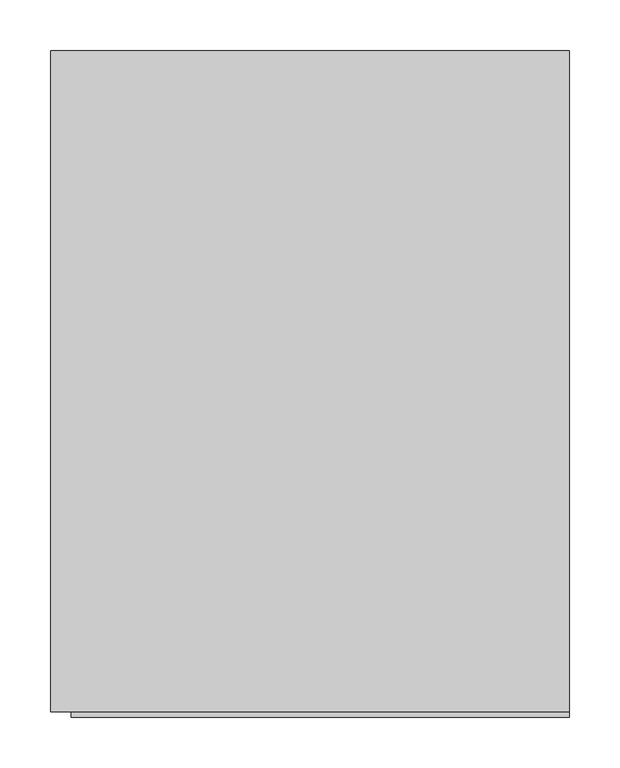
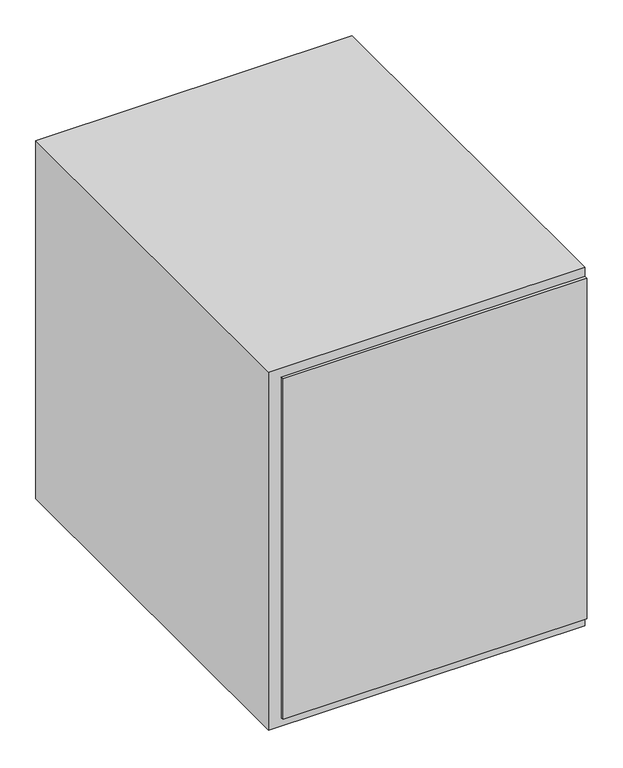
"""IFC4 building model written with IfcOpenShell, lengths in millimetres: proxy geometry, Тропик-30 : LNVx 45F."""

from ifc_helpers import new_model, si_unit, frame, origin, origin_with_axes, place, context, project, spatial, polyline, outline, extrude, source, transform, mapped, element, save


def mechanical_equipment_ab37a4de(model_context):
    return source(origin(), model_context, "Body", "SweptSolid", [
        extrude(outline(polyline([(255.0, -330.0), (-234.7800933, -330.0), (-234.7800933, -325.0), (255.0, -325.0), (255.0, -330.0)])), frame((0.0, 0.0, 14.5270889), z_axis=(0.0, 0.0, 1.0), x_axis=(1.0, 0.0, 0.0)), (0.0, 0.0, 1.0), 580.0),
        extrude(outline(polyline([(255.0, 325.0), (255.0, -325.0), (-255.0, -325.0), (-255.0, 325.0), (255.0, 325.0)])), origin_with_axes(), (0.0, 0.0, 1.0), 610.0),
    ])


if __name__ == "__main__":
    model = new_model("IFC4")
    model_context = context("Model", 3, world=origin())
    ifc_project = project(units=[si_unit("LENGTHUNIT", "METRE", prefix="MILLI")], contexts=[model_context])
    site = spatial("IfcSite", under=ifc_project)
    building = spatial("IfcBuilding", under=site)
    placement = place(None, origin())
    mechanical_equipment_shape = mechanical_equipment_ab37a4de(model_context)
    element("IfcBuildingElementProxy", 1, Name="Тропик-30 : LNVx 45F", ObjectType="Тропик-30 : LNVx 45F", at=placement, inside=building, context=model_context, shape_type="MappedRepresentation", body=[
        mapped(mechanical_equipment_shape, transform((0.0, 0.0, 0.0), x_axis=(1.0, 0.0, 0.0), y_axis=(0.0, 1.0, 0.0), z_axis=(0.0, 0.0, 1.0))),
    ])
    save(model, "model.ifc")

# Revit data of these elements
# Type "Тропик-30 : LNVx 45F"
#   ADSK_Наименование = "Тепловентилятор\"Тропик\" с мощностью 3 кВт"
#   Width = 650 mm
#   Length = 510 mm
#   Height = 610 mm
#   Material = RAL 7015
#   Default Elevation = 0
#   Manufacturer = ""
#   Description = (empty or 0)
# Element 1 (IfcBuildingElementProxy, "Тропик-30 : LNVx 45F")
#   Materials on its faces: "RAL 7015"
# Materials
#   "RAL 7015": class "Generic", colour RGB 120 120 120, transparency 0, Cost = 0
